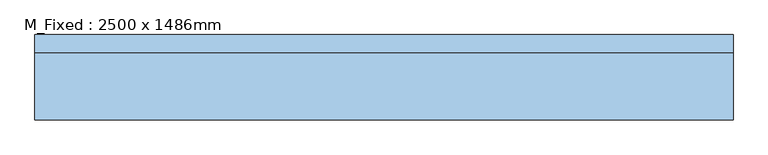
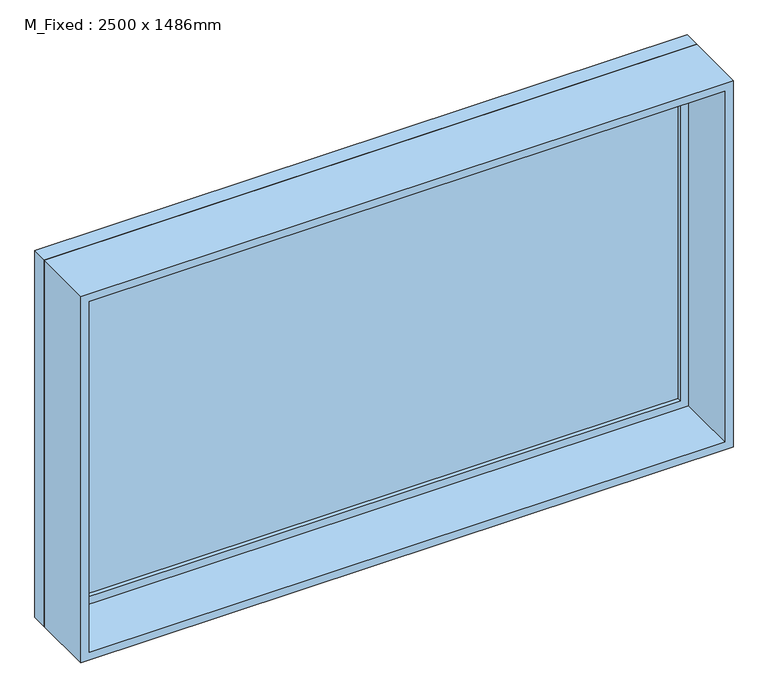
"""IFC4 building model written with IfcOpenShell, lengths in millimetres: window geometry, M_Fixed : 2500 x 1486mm."""

from ifc_helpers import new_model, si_unit, frame, origin, place, context, project, spatial, polyline, outline, extrude, source, transform, mapped, element, save


def m_fixed_2500_x_1486mm_baf7df51(model_context):
    return source(origin(), model_context, "Body", "SweptSolid", [
        extrude(outline(polyline([(-1187.0, 130.4), (1187.0, 130.4), (1187.0, 118.4), (-1187.0, 118.4), (-1187.0, 130.4)])), frame((0.0, 0.0, 978.0), z_axis=(0.0, 0.0, 1.0), x_axis=(1.0, 0.0, 0.0)), (0.0, 0.0, 1.0), 1360.5),
        extrude(outline(polyline([(2382.5, -1231.0), (934.0, -1231.0), (934.0, 1231.0), (2382.5, 1231.0), (2382.5, -1231.0)]), holes=[polyline([(2338.5, -1187.0), (2338.5, 1187.0), (978.0, 1187.0), (978.0, -1187.0), (2338.5, -1187.0)])]), frame((0.0, 102.4, 0.0), z_axis=(0.0, 1.0, 0.0), x_axis=(0.0, 0.0, 1.0)), (0.0, 0.0, 1.0), 44.0),
        extrude(outline(polyline([(2401.5, -1250.0), (915.0, -1250.0), (915.0, 1250.0), (2401.5, 1250.0), (2401.5, -1250.0)]), holes=[polyline([(2382.5, -1231.0), (2382.5, 1231.0), (934.0, 1231.0), (934.0, -1231.0), (2382.5, -1231.0)])]), frame((0.0, 102.4, 0.0), z_axis=(0.0, 1.0, 0.0), x_axis=(0.0, 0.0, 1.0)), (0.0, 0.0, 1.0), 63.0),
        extrude(outline(polyline([(2401.5, -1250.0), (915.0, -1250.0), (915.0, 1250.0), (2401.5, 1250.0), (2401.5, -1250.0)]), holes=[polyline([(2369.5, -1218.0), (2369.5, 1218.0), (947.0, 1218.0), (947.0, -1218.0), (2369.5, -1218.0)])]), frame((0.0, -139.4, 0.0), z_axis=(0.0, 1.0, 0.0), x_axis=(0.0, 0.0, 1.0)), (0.0, 0.0, 1.0), 241.8),
    ])


if __name__ == "__main__":
    model = new_model("IFC4")
    model_context = context("Model", 3, world=origin())
    ifc_project = project(units=[si_unit("LENGTHUNIT", "METRE", prefix="MILLI")], contexts=[model_context])
    site = spatial("IfcSite", under=ifc_project)
    building = spatial("IfcBuilding", under=site)
    placement = place(None, origin())
    m_fixed_2500_x_1486mm_shape = m_fixed_2500_x_1486mm_baf7df51(model_context)
    element("IfcWindow", 1, ObjectType="M_Fixed : 2500 x 1486mm", at=placement, inside=building, context=model_context, shape_type="MappedRepresentation", body=[
        mapped(m_fixed_2500_x_1486mm_shape, transform((0.0, 0.0, 0.0), x_axis=(1.0, 0.0, 0.0), y_axis=(0.0, 1.0, 0.0), z_axis=(0.0, 0.0, 1.0))),
    ])
    save(model, "model.ifc")

# Revit data of these elements
# Type "M_Fixed : 2500 x 1486mm"
#   Type Mark = "19"
#   Height = 1486.5 mm
#   Default Sill Height = 915 mm
#   Width = 2500 mm
#   Window Inset = 19 mm
#   Frame Exterior Material = Sash
#   Frame Interior Material = Sash
#   Glass Pane Material = Glass
#   Sash = Sash
#   Wall Closure = (empty or 0)
# Element 1 (IfcWindow, "M_Fixed : 2500 x 1486mm")
#   Materials on its faces: "Sash", "Glass"
# Materials
#   "Sash": class "Wood", colour RGB 136 99 55, transparency 0
#   "Glass": class "Glass", colour RGB 0 128 192, transparency 0.9, Description = "Soda Lime Glass", Cost = 0
